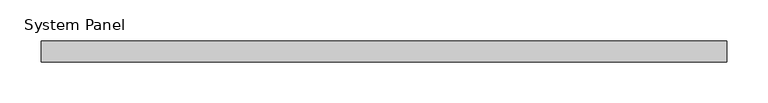
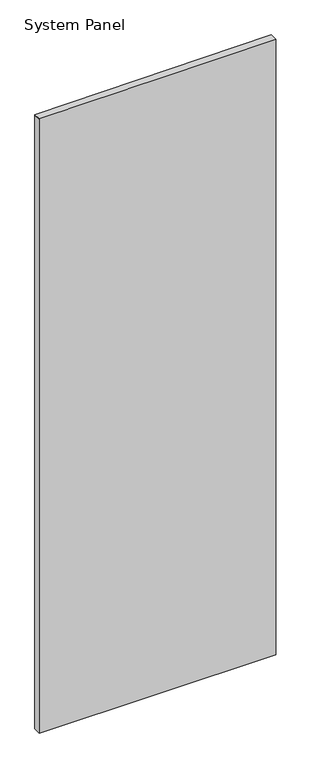
"""IFC4 building model written with IfcOpenShell, lengths in millimetres: plate geometry, System Panel : TEMPERED INSULATED GLAZING (CARDINAL GLASS LoĒ²-240."""

from ifc_helpers import new_model, si_unit, frame, origin, place, context, project, spatial, polyline, outline, extrude, source, transform, mapped, element, save


def system_panel_df04ebb9(model_context):
    return source(origin(), model_context, "Body", "SweptSolid", [
        extrude(outline(polyline([(0.0, -416.8619325), (0.0, 416.8619325), (2287.5080968, 416.8619325), (2294.3902848, 416.8619325), (2289.0265376, -416.8619325), (2287.5080968, -416.8619325), (0.0, -416.8619325)])), frame((0.0, -31.75, 0.0), z_axis=(0.0, 1.0, 0.0), x_axis=(0.0, 0.0, 1.0)), (0.0, 0.0, 1.0), 25.4),
    ])


if __name__ == "__main__":
    model = new_model("IFC4")
    model_context = context("Model", 3, world=origin())
    ifc_project = project(units=[si_unit("LENGTHUNIT", "METRE", prefix="MILLI")], contexts=[model_context])
    site = spatial("IfcSite", under=ifc_project)
    building = spatial("IfcBuilding", under=site)
    placement = place(None, origin())
    system_panel_shape = system_panel_df04ebb9(model_context)
    element("IfcPlate", 1, ObjectType="System Panel : TEMPERED INSULATED GLAZING (CARDINAL GLASS LoĒ²-240", at=placement, inside=building, context=model_context, shape_type="MappedRepresentation", body=[
        mapped(system_panel_shape, transform((0.0, 0.0, 0.0), x_axis=(1.0, 0.0, 0.0), y_axis=(0.0, 1.0, 0.0), z_axis=(0.0, 0.0, 1.0))),
    ])
    save(model, "model.ifc")

# Revit data of these elements
# Type "System Panel : TEMPERED INSULATED GLAZING (CARDINAL GLASS LoĒ²-240"
#   Construction Type Id = "opn-s72"
#   Analytic Construction = "Double glazing - 1/4 in thick - low-E/clear (e = 0.1) glass"
#   Visual Light Transmittance = 0.72
#   Solar Heat Gain Coefficient = 0.6
#   Heat Transfer Coefficient (U) = 1.9873 W/(m²·K)
#   Transparency_Hack = 70
# Element 1 (IfcPlate, "System Panel : TEMPERED INSULATED GLAZING (CARDINAL GLASS LoĒ²-240")
#   Materials on its faces: "TEMPERED INSULATED GLAZING (CARDINAL GLASS LoĒ²-240\nOR EQUIVALENT)"
# Materials
#   "TEMPERED INSULATED GLAZING (CARDINAL GLASS LoĒ²-240\nOR EQUIVALENT)": class "Glass", colour RGB 196 205 210, transparency 0.85, Description = "Soda Lime Glass", Cost = 0
